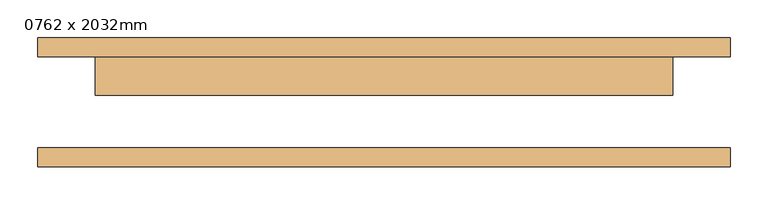
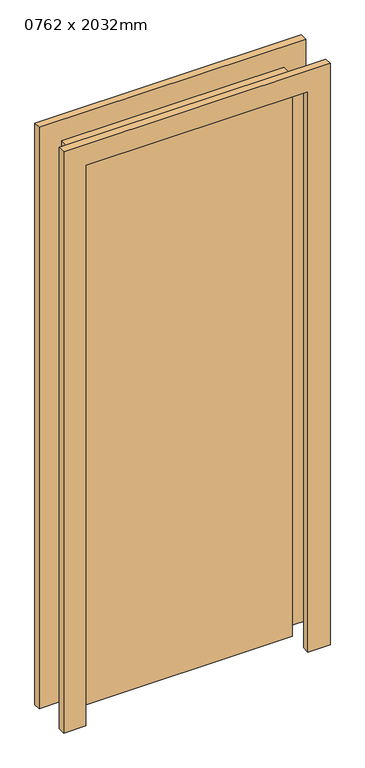
"""IFC4 building model written with IfcOpenShell, lengths in millimetres: door geometry, M_Folha única : 0762 x 2032mm."""

from ifc_helpers import new_model, si_unit, frame, origin, origin_with_axes, place, context, project, spatial, polyline, outline, extrude, source, transform, mapped, element, save


def door_0762_x_2032mm_ca16c8eb(model_context):
    return source(origin(), model_context, "Body", "SweptSolid", [
        extrude(outline(polyline([(2108.0, -457.0), (0.0, -457.0), (0.0, -381.0), (2032.0, -381.0), (2032.0, 381.0), (0.0, 381.0), (0.0, 457.0), (2108.0, 457.0), (2108.0, -457.0)])), frame((0.0, 60.0, 0.0), z_axis=(0.0, 1.0, 0.0), x_axis=(0.0, 0.0, 1.0)), (0.0, 0.0, 1.0), 25.0),
        extrude(outline(polyline([(2108.0, 457.0), (2108.0, -457.0), (0.0, -457.0), (0.0, -381.0), (2032.0, -381.0), (2032.0, 381.0), (0.0, 381.0), (0.0, 457.0), (2108.0, 457.0)])), frame((0.0, -85.0, 0.0), z_axis=(0.0, 1.0, 0.0), x_axis=(0.0, 0.0, 1.0)), (0.0, 0.0, 1.0), 25.0),
        extrude(outline(polyline([(381.0, 9.0), (-381.0, 9.0), (-381.0, 60.0), (381.0, 60.0), (381.0, 9.0)])), origin_with_axes(), (0.0, 0.0, 1.0), 2032.0),
    ])


if __name__ == "__main__":
    model = new_model("IFC4")
    model_context = context("Model", 3, world=origin())
    ifc_project = project(units=[si_unit("LENGTHUNIT", "METRE", prefix="MILLI")], contexts=[model_context])
    site = spatial("IfcSite", under=ifc_project)
    building = spatial("IfcBuilding", under=site)
    placement = place(None, origin())
    door_0762_x_2032mm_shape = door_0762_x_2032mm_ca16c8eb(model_context)
    element("IfcDoor", 1, ObjectType="M_Folha única : 0762 x 2032mm", at=placement, inside=building, context=model_context, shape_type="MappedRepresentation", body=[
        mapped(door_0762_x_2032mm_shape, transform((0.0, 0.0, 0.0), x_axis=(1.0, 0.0, 0.0), y_axis=(0.0, 1.0, 0.0), z_axis=(0.0, 0.0, 1.0))),
    ])
    save(model, "model.ifc")

# Revit data of these elements
# Type "M_Folha única : 0762 x 2032mm"
#   Type Mark = "28"
#   Construction Type Id = "MDOOR"
#   Analytic Construction = "Metal"
#   Thickness = 0.051 m
#   Thermal Resistance (R) = 0.270117 (m²·K)/W
#   Heat Transfer Coefficient (U) = 3.7021 W/(m²·K)
#   Height = 2.032 m
#   Projeção da apara externa = 0.025 m
#   Projeção da apara interna = 0.025 m
#   Largura da apara = 0.076 m
#   Width = 0.762 m
#   Define Thermal Properties by = 1
#   Define Thermal Properties by = 1
#   Material da porta = Porta - Painel
#   Material da moldura = Porta - Batente
#   Visual Light Transmittance = 0
#   Solar Heat Gain Coefficient = 0
#   Function = (empty or 0)
#   Wall Closure = (empty or 0)
# Element 1 (IfcDoor, "M_Folha única : 0762 x 2032mm")
#   Materials on its faces: "Porta - Batente", "Porta - Painel"
# Materials
#   "Porta - Painel": class "Madeira", colour RGB 210 159 95, transparency 0, Cost = 0
#   "Porta - Batente": class "Diversos", colour RGB 118 70 51, transparency 0, Cost = 0
